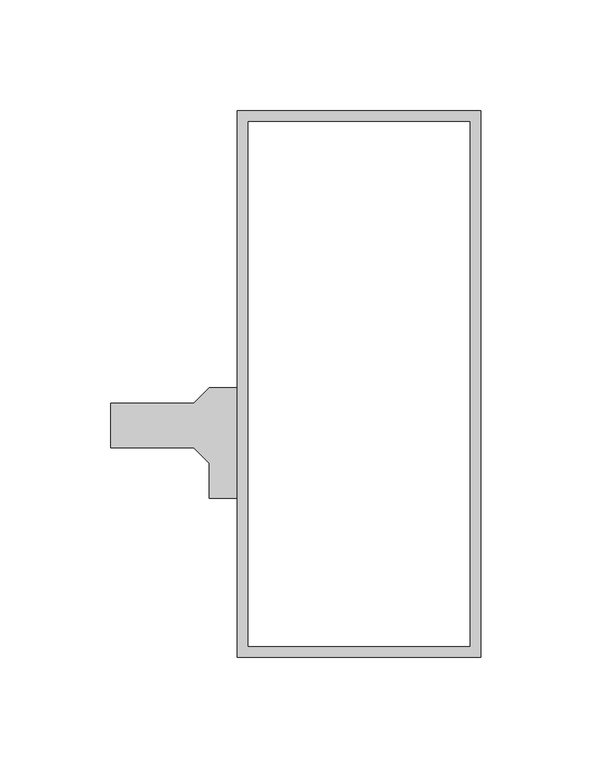
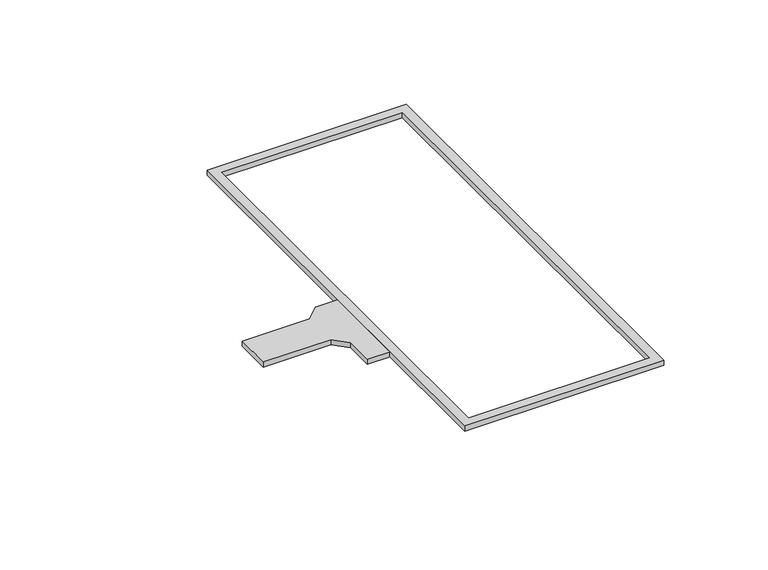
"""IFC4 building model written with IfcOpenShell, lengths in millimetres: proxy geometry, TSP Braai LightPoint : TSP Braai LightPoint."""

from ifc_helpers import new_model, si_unit, origin, origin_with_axes, place, context, project, spatial, polyline, outline, extrude, source, transform, mapped, element, save


def electrical_fixtures_1e9f52fa(model_context):
    return source(origin(), model_context, "Body", "SweptSolid", [
        extrude(outline(polyline([(105.0, 125.0229032), (105.0, -121.6770968), (-5.0, -121.6770968), (-5.0, 125.0229032), (105.0, 125.0229032)]), holes=[polyline([(100.0, 120.0229032), (0.0, 120.0229032), (0.0, -116.6770968), (100.0, -116.6770968), (100.0, 120.0229032)])]), origin_with_axes(), (0.0, 0.0, 1.0), 3.0),
        extrude(outline(polyline([(-17.5, 0.0), (-5.0, 0.0), (-5.0, -50.0), (-17.5, -50.0), (-17.5, -34.1421356), (-24.5710678, -27.0710678), (-62.0710678, -27.0710678), (-62.0710678, -7.0710678), (-24.5710678, -7.0710678), (-17.5, 0.0)])), origin_with_axes(), (0.0, 0.0, 1.0), 3.0),
    ])


if __name__ == "__main__":
    model = new_model("IFC4")
    model_context = context("Model", 3, world=origin())
    ifc_project = project(units=[si_unit("LENGTHUNIT", "METRE", prefix="MILLI")], contexts=[model_context])
    site = spatial("IfcSite", under=ifc_project)
    building = spatial("IfcBuilding", under=site)
    placement = place(None, origin())
    electrical_fixtures_shape = electrical_fixtures_1e9f52fa(model_context)
    element("IfcBuildingElementProxy", 1, Name="TSP Braai LightPoint : TSP Braai LightPoint", ObjectType="TSP Braai LightPoint : TSP Braai LightPoint", at=placement, inside=building, context=model_context, shape_type="MappedRepresentation", body=[
        mapped(electrical_fixtures_shape, transform((0.0, 0.0, 0.0), x_axis=(1.0, 0.0, 0.0), y_axis=(0.0, 1.0, 0.0), z_axis=(0.0, 0.0, 1.0))),
    ])
    save(model, "model.ifc")

# Revit data of these elements
# Type "TSP Braai LightPoint : TSP Braai LightPoint"
#   Model = "TSP_ELEC220BLP"
#   Default Elevation = 0
# Element 1 (IfcBuildingElementProxy, "TSP Braai LightPoint : TSP Braai LightPoint")
#   Materials on its faces: "Plastic, Opaque Black"
# Materials
#   "Plastic, Opaque Black": class "Plastic", colour RGB 0 0 0, transparency 0.7, Description = "Plastic, generic, opaque black", Cost = 0
